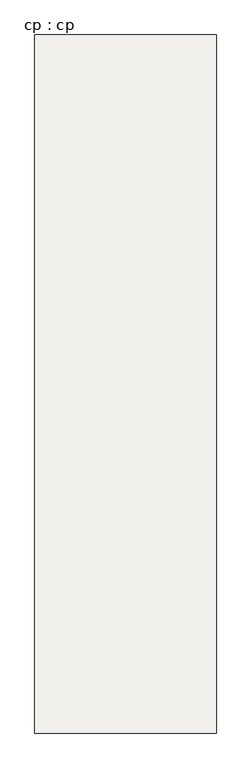
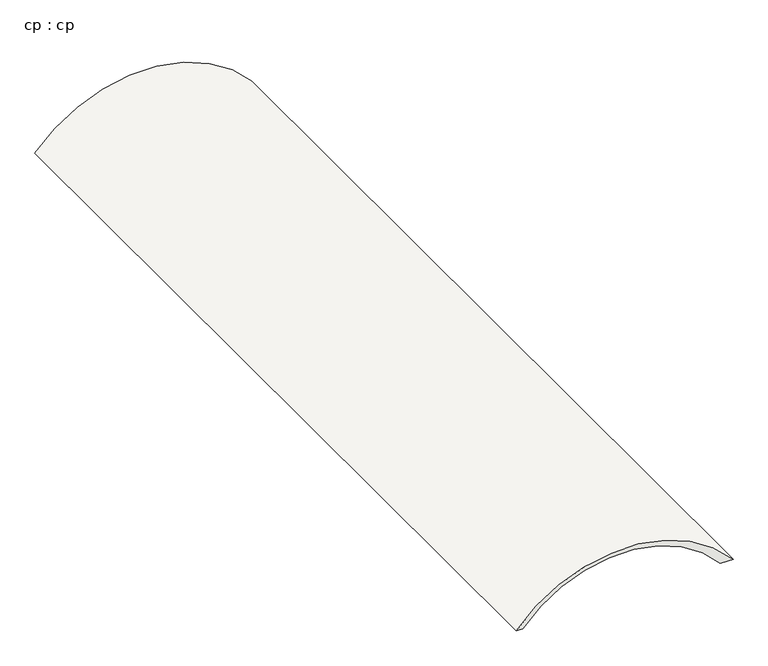
"""IFC4 building model written with IfcOpenShell, lengths in millimetres: slab geometry, cp : cp."""

from ifc_helpers import new_model, si_unit, point, frame, frame_2d, origin, place, context, project, spatial, polyline, circle_curve, trimmed, segment, composite_curve, outline, extrude, source, transform, mapped, element, save


def cp_cp_a82b7de9(model_context):
    return source(origin(), model_context, "Body", "SweptSolid", [
        extrude(outline(composite_curve([segment(polyline([(14620.0, 50183.2245511), (14620.0, 50483.2245511)]), True, "CONTINUOUS"), segment(trimmed(circle_curve(frame_2d((12402.7966102, 47908.2245512)), 3398.0311757), [point((14620.0, 50483.2245511))], [point((14620.0, 45333.2245512))], False, "CARTESIAN"), True, "CONTINUOUS"), segment(polyline([(14620.0, 45333.2245512), (14620.0, 45483.2245512)]), True, "CONTINUOUS"), segment(trimmed(circle_curve(frame_2d((12608.2612414, 47833.2245512)), 3093.4758497), [point((14620.0, 45483.2245512))], [point((14620.0, 50183.2245511))], True, "CARTESIAN"), True, "CONTINUOUS")], self_intersect=False)), frame((0.0, -100.2551788, 0.0), z_axis=(0.0, 1.0, 0.0), x_axis=(0.0, 0.0, 1.0)), (0.0, 0.0, 1.0), 19800.2551781),
    ])


if __name__ == "__main__":
    model = new_model("IFC4")
    model_context = context("Model", 3, world=origin())
    ifc_project = project(units=[si_unit("LENGTHUNIT", "METRE", prefix="MILLI")], contexts=[model_context])
    site = spatial("IfcSite", under=ifc_project)
    building = spatial("IfcBuilding", under=site)
    placement = place(None, origin())
    cp_cp_shape = cp_cp_a82b7de9(model_context)
    element("IfcSlab", 1, ObjectType="cp : cp", at=placement, inside=building, context=model_context, shape_type="MappedRepresentation", body=[
        mapped(cp_cp_shape, transform((0.0, 0.0, 0.0), x_axis=(1.0, 0.0, 0.0), y_axis=(0.0, 1.0, 0.0), z_axis=(0.0, 0.0, 1.0))),
    ])
    save(model, "model.ifc")

# Revit data of these elements
# Type "cp : cp"
#   Structural Material = Concrete, RC
# Element 1 (IfcSlab, "cp : cp")
#   Materials on its faces: "Concrete, RC"
# Materials
#   "Concrete, RC": class "Concrete", colour RGB 128 128 128, transparency 0, Description = "Cast-in-place concrete", Cost = 0
